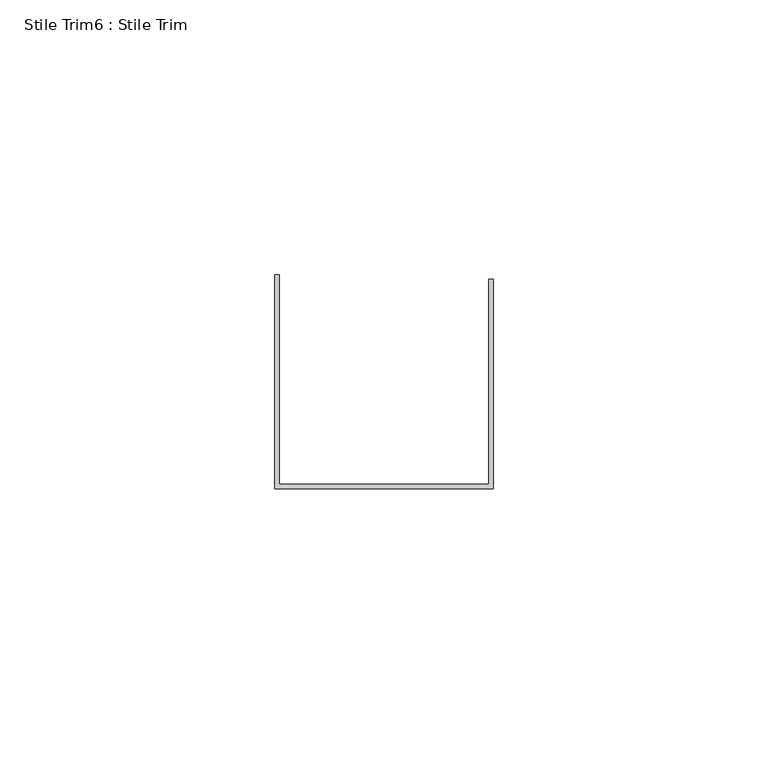
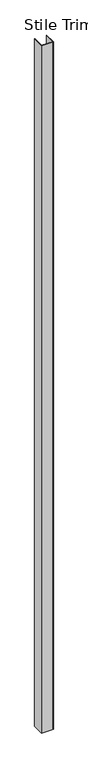
"""IFC4 building model written with IfcOpenShell, lengths in millimetres: proxy geometry, Stile Trim6 : Stile Trim."""

import ifcopenshell
import ifcopenshell.guid

model = None  # the IFC model being written
_history = None  # IfcOwnerHistory: only IFC2X3 demands one
_inside = {}  # id of a spatial element -> (the spatial element, [elements in it])
_under = {}  # id of a project, library or spatial element -> (it, [spatial elements below it])
_declared = {}  # id of a project -> (the project, [libraries it declares])
_typed = {}  # id of a type object -> (the type object, [elements of that type])
_made_of = {}  # id of a material, layer set ... -> (it, [elements and type objects made of it])


def new_model(schema):
    """Start an empty IFC model of exactly this schema.

    Asked for "IFC4X3", IfcOpenShell would pick the latest addendum, in which some entities
    have other attributes; the version numbers below select the first issue.
    IFC2X3 requires an IfcOwnerHistory on every rooted entity: one is made here for all.
    """
    global model, _history
    if schema == "IFC4X3":
        model = ifcopenshell.file(schema_version=(4, 3, 0, 0))
    else:
        model = ifcopenshell.file(schema=schema)
    _inside.clear()
    _under.clear()
    _declared.clear()
    _typed.clear()
    _made_of.clear()
    _history = None
    if model.schema == "IFC2X3":
        org = make("IfcOrganization", Name="unknown")
        user = make(
            "IfcPersonAndOrganization",
            ThePerson=make("IfcPerson", FamilyName="unknown"),
            TheOrganization=org,
        )
        app = make(
            "IfcApplication",
            ApplicationDeveloper=org,
            Version="unknown",
            ApplicationFullName="unknown",
            ApplicationIdentifier="unknown",
        )
        _history = make(
            "IfcOwnerHistory",
            OwningUser=user,
            OwningApplication=app,
            ChangeAction="ADDED",
            CreationDate=0,
        )
    return model


def make(cls, **values):
    """One entity of the class cls with the attributes given. An attribute that is None is left unset."""
    return model.create_entity(
        cls, **{name: value for name, value in values.items() if value is not None}
    )


def rooted(cls, **values):
    """An entity with a GlobalId (a new one), such as an element, a storey or a relation."""
    return make(cls, GlobalId=ifcopenshell.guid.new(), OwnerHistory=_history, **values)


def si_unit(unit_type, name, prefix=None):
    """IfcSIUnit, for example si_unit("LENGTHUNIT", "METRE", prefix="MILLI")."""
    return make("IfcSIUnit", UnitType=unit_type, Prefix=prefix, Name=name)


def assignment(units):
    """IfcUnitAssignment: the units of a project."""
    return None if units is None else make("IfcUnitAssignment", Units=units)


def point(xyz):
    """IfcCartesianPoint."""
    return None if xyz is None else make("IfcCartesianPoint", Coordinates=xyz)


def direction(xyz):
    """IfcDirection."""
    return None if xyz is None else make("IfcDirection", DirectionRatios=xyz)


def frame(location, z_axis=None, x_axis=None):
    """IfcAxis2Placement3D, a coordinate frame: its origin and axes. An axis left out is left unset."""
    return make(
        "IfcAxis2Placement3D",
        Location=point(location),
        Axis=direction(z_axis),
        RefDirection=direction(x_axis),
    )


def origin():
    """The frame at (0, 0, 0) with its axes left unset."""
    return frame((0.0, 0.0, 0.0))


def place(relative_to, where):
    """IfcLocalPlacement: puts the frame where relative to a parent placement (None: the world)."""
    return make(
        "IfcLocalPlacement", PlacementRelTo=relative_to, RelativePlacement=where
    )


def context(
    kind, dimensions, precision=None, world=None, true_north=None, identifier=None
):
    """IfcGeometricRepresentationContext, for example the 3D "Model" context."""
    return make(
        "IfcGeometricRepresentationContext",
        ContextIdentifier=identifier,
        ContextType=kind,
        CoordinateSpaceDimension=dimensions,
        Precision=precision,
        WorldCoordinateSystem=world,
        TrueNorth=true_north,
    )


def project(units=None, contexts=None):
    """IfcProject with its units and contexts."""
    return rooted(
        "IfcProject",
        Name="project",
        RepresentationContexts=contexts,
        UnitsInContext=assignment(units),
    )


def spatial(cls, under=None, at=None, **own):
    """A site, building, storey or space (cls), placed at a placement, below another one or the project."""
    s = rooted(cls, ObjectPlacement=at, **own)
    if under is not None:
        _under.setdefault(under.id(), (under, []))[1].append(s)
    return s


def polyline(points):
    """IfcPolyline through the points."""
    return make("IfcPolyline", Points=[point(p) for p in points])


def outline(outer, holes=None, kind="AREA"):
    """IfcArbitraryClosedProfileDef: a profile drawn as a closed curve; with holes, ...WithVoids."""
    if holes is None:
        return make("IfcArbitraryClosedProfileDef", ProfileType=kind, OuterCurve=outer)
    return make(
        "IfcArbitraryProfileDefWithVoids",
        ProfileType=kind,
        OuterCurve=outer,
        InnerCurves=holes,
    )


def extrude(swept, where, along, depth):
    """IfcExtrudedAreaSolid: the profile swept, set in the frame where, extruded along a direction by depth."""
    return make(
        "IfcExtrudedAreaSolid",
        SweptArea=swept,
        Position=where,
        ExtrudedDirection=direction(along),
        Depth=depth,
    )


def shape(context_of_items, identifier, shape_type, items):
    """IfcShapeRepresentation: the items that make up one representation, for example the "Body"."""
    return make(
        "IfcShapeRepresentation",
        ContextOfItems=context_of_items,
        RepresentationIdentifier=identifier,
        RepresentationType=shape_type,
        Items=items,
    )


def source(mapping_origin, context_of_items, identifier, shape_type, items):
    """IfcRepresentationMap: a shape defined once, which mapped items show again and again."""
    return make(
        "IfcRepresentationMap",
        MappingOrigin=mapping_origin,
        MappedRepresentation=shape(context_of_items, identifier, shape_type, items),
    )


def transform(
    local_origin,
    x_axis=None,
    y_axis=None,
    z_axis=None,
    scale=None,
    scale2=None,
    scale3=None,
    uniform=True,
):
    """IfcCartesianTransformationOperator3D, or its non-uniform kind. x_axis, y_axis, z_axis: its Axis1, 2, 3."""
    if uniform:
        return make(
            "IfcCartesianTransformationOperator3D",
            Axis1=direction(x_axis),
            Axis2=direction(y_axis),
            LocalOrigin=point(local_origin),
            Scale=scale,
            Axis3=direction(z_axis),
        )
    return make(
        "IfcCartesianTransformationOperator3DnonUniform",
        Axis1=direction(x_axis),
        Axis2=direction(y_axis),
        LocalOrigin=point(local_origin),
        Scale=scale,
        Axis3=direction(z_axis),
        Scale2=scale2,
        Scale3=scale3,
    )


def mapped(mapping_source, mapping_target):
    """IfcMappedItem: shows the shape of a source again, moved by a transform."""
    return make(
        "IfcMappedItem", MappingSource=mapping_source, MappingTarget=mapping_target
    )


def made_of(thing, what):
    """Note that an element or type object is made of a material, layer set ...; save() writes the relation."""
    if what is not None:
        _made_of.setdefault(what.id(), (what, []))[1].append(thing)
    return thing


def element(
    cls,
    number,
    at=None,
    inside=None,
    cuts=None,
    type_object=None,
    material=None,
    context=None,
    identifier="Body",
    shape_type=None,
    held_by="IfcProductDefinitionShape",
    body=None,
    shapes=None,
    **own,
):
    """One element of the class cls, such as IfcWall. Its Tag is "e" and its number.

    at: its placement. inside: the storey or other place that contains it. cuts: it is an
    opening in that element (IfcRelVoidsElement). A single representation is given by context,
    identifier, shape_type and body (its items); several are given by shapes. held_by: the class
    of the entity that holds the representations. save() writes the other relations.
    """
    e = rooted(cls, Tag="e%d" % number, ObjectPlacement=at, **own)
    if body is not None:
        shapes = [shape(context, identifier, shape_type, body)]
    if shapes is not None:
        e.Representation = make(held_by, Representations=shapes)
    if inside is not None:
        _inside.setdefault(inside.id(), (inside, []))[1].append(e)
    if cuts is not None:
        rooted(
            "IfcRelVoidsElement", RelatingBuildingElement=cuts, RelatedOpeningElement=e
        )
    if type_object is not None:
        _typed.setdefault(type_object.id(), (type_object, []))[1].append(e)
    return made_of(e, material)


def aggregate(whole, parts):
    """IfcRelAggregates: a whole, such as a stair, and the parts it consists of."""
    return rooted("IfcRelAggregates", RelatingObject=whole, RelatedObjects=parts)


def save(model, path):
    """Write the relations noted so far, then the file.

    IfcRelAggregates (storeys below a building ...), IfcRelContainedInSpatialStructure (elements
    in a storey), IfcRelDefinesByType, IfcRelAssociatesMaterial and IfcRelDeclares: one each for
    every whole, place, type object, material and project.
    """
    for whole, parts in _under.values():
        aggregate(whole, parts)
    for where, things in _inside.values():
        rooted(
            "IfcRelContainedInSpatialStructure",
            RelatedElements=things,
            RelatingStructure=where,
        )
    for kind, things in _typed.values():
        rooted("IfcRelDefinesByType", RelatedObjects=things, RelatingType=kind)
    for what, things in _made_of.values():
        rooted("IfcRelAssociatesMaterial", RelatedObjects=things, RelatingMaterial=what)
    for by, libraries in _declared.values():
        rooted("IfcRelDeclares", RelatingContext=by, RelatedDefinitions=libraries)
    model.write(path)


def stile_trim6_stile_trim_7538b4aa(model_context):
    return source(origin(), model_context, "Body", "SweptSolid", [
        extrude(outline(polyline([(587327.0060739, -531776.5287841), (587327.0060739, -531737.6413841), (587327.7934739, -531737.6413841), (587327.7934739, -531775.7413841), (587365.8934739, -531775.7413841), (587365.8934739, -531738.4287841), (587366.6808739, -531738.4287841), (587366.6808739, -531776.5287841), (587327.0060739, -531776.5287841)])), frame((0.0, 0.0, 11.90625), z_axis=(0.0, 0.0, 1.0), x_axis=(1.0, 0.0, 0.0)), (0.0, 0.0, 1.0), 2426.49375),
    ])


if __name__ == "__main__":
    model = new_model("IFC4")
    model_context = context("Model", 3, world=origin())
    ifc_project = project(units=[si_unit("LENGTHUNIT", "METRE", prefix="MILLI")], contexts=[model_context])
    site = spatial("IfcSite", under=ifc_project)
    building = spatial("IfcBuilding", under=site)
    placement = place(None, origin())
    stile_trim6_stile_trim_shape = stile_trim6_stile_trim_7538b4aa(model_context)
    element("IfcBuildingElementProxy", 1, Name="Stile Trim6 : Stile Trim", ObjectType="Stile Trim6 : Stile Trim", at=placement, inside=building, context=model_context, shape_type="MappedRepresentation", body=[
        mapped(stile_trim6_stile_trim_shape, transform((0.0, 0.0, 0.0), x_axis=(1.0, 0.0, 0.0), y_axis=(0.0, 1.0, 0.0), z_axis=(0.0, 0.0, 1.0))),
    ])
    save(model, "model.ifc")

# Revit data of these elements
# Element 1 (IfcBuildingElementProxy, "Stile Trim6 : Stile Trim")
#   Materials on its faces: "EDGE TRIM BY MTL PANEL MFR."
# Materials
#   "EDGE TRIM BY MTL PANEL MFR.": class "Generic", colour RGB 239 242 240, transparency 0, Cost = 0
